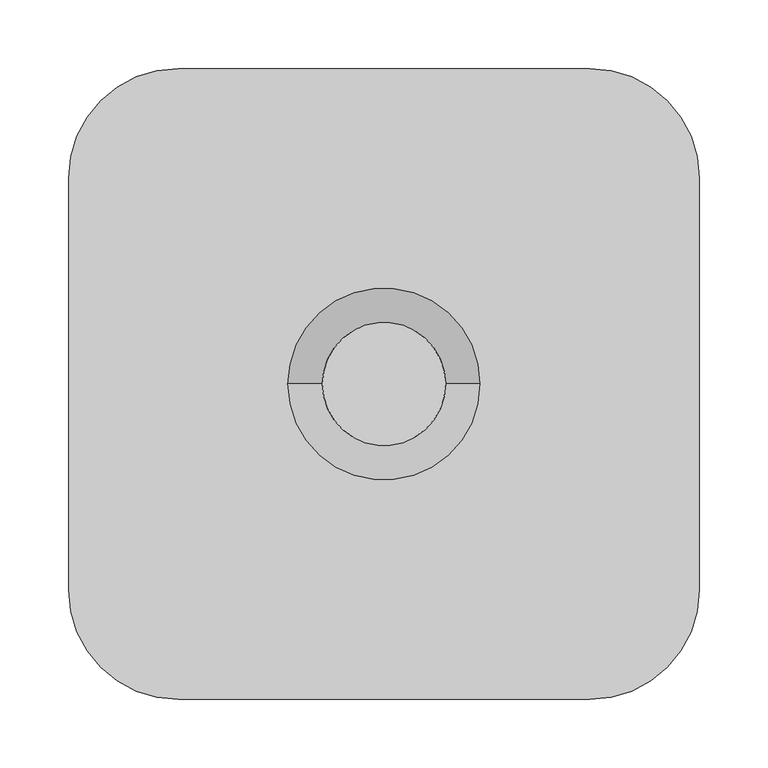
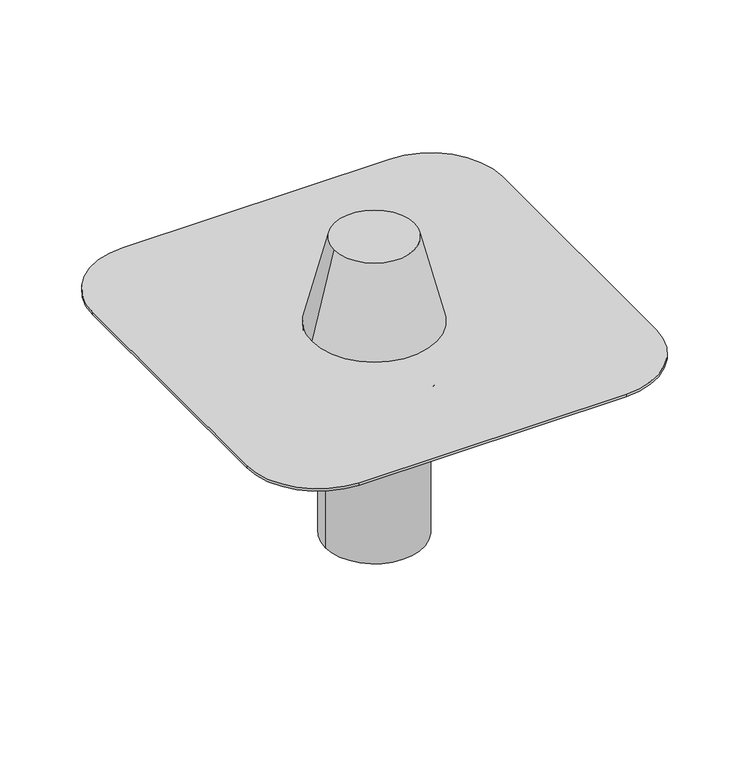
"""IFC4 building model written with IfcOpenShell, lengths in millimetres: proxy geometry, TN_ПВХ Воронка экструдированная с листоуловителем : ПВХ Воронка экструдированная 110х240мм с листоуловителем."""

import ifcopenshell
import ifcopenshell.guid

model = None  # the IFC model being written
_history = None  # IfcOwnerHistory: only IFC2X3 demands one
_inside = {}  # id of a spatial element -> (the spatial element, [elements in it])
_under = {}  # id of a project, library or spatial element -> (it, [spatial elements below it])
_declared = {}  # id of a project -> (the project, [libraries it declares])
_typed = {}  # id of a type object -> (the type object, [elements of that type])
_made_of = {}  # id of a material, layer set ... -> (it, [elements and type objects made of it])


def new_model(schema):
    """Start an empty IFC model of exactly this schema.

    Asked for "IFC4X3", IfcOpenShell would pick the latest addendum, in which some entities
    have other attributes; the version numbers below select the first issue.
    IFC2X3 requires an IfcOwnerHistory on every rooted entity: one is made here for all.
    """
    global model, _history
    if schema == "IFC4X3":
        model = ifcopenshell.file(schema_version=(4, 3, 0, 0))
    else:
        model = ifcopenshell.file(schema=schema)
    _inside.clear()
    _under.clear()
    _declared.clear()
    _typed.clear()
    _made_of.clear()
    _history = None
    if model.schema == "IFC2X3":
        org = make("IfcOrganization", Name="unknown")
        user = make(
            "IfcPersonAndOrganization",
            ThePerson=make("IfcPerson", FamilyName="unknown"),
            TheOrganization=org,
        )
        app = make(
            "IfcApplication",
            ApplicationDeveloper=org,
            Version="unknown",
            ApplicationFullName="unknown",
            ApplicationIdentifier="unknown",
        )
        _history = make(
            "IfcOwnerHistory",
            OwningUser=user,
            OwningApplication=app,
            ChangeAction="ADDED",
            CreationDate=0,
        )
    return model


def make(cls, **values):
    """One entity of the class cls with the attributes given. An attribute that is None is left unset."""
    return model.create_entity(
        cls, **{name: value for name, value in values.items() if value is not None}
    )


def rooted(cls, **values):
    """An entity with a GlobalId (a new one), such as an element, a storey or a relation."""
    return make(cls, GlobalId=ifcopenshell.guid.new(), OwnerHistory=_history, **values)


def si_unit(unit_type, name, prefix=None):
    """IfcSIUnit, for example si_unit("LENGTHUNIT", "METRE", prefix="MILLI")."""
    return make("IfcSIUnit", UnitType=unit_type, Prefix=prefix, Name=name)


def assignment(units):
    """IfcUnitAssignment: the units of a project."""
    return None if units is None else make("IfcUnitAssignment", Units=units)


def point(xyz):
    """IfcCartesianPoint."""
    return None if xyz is None else make("IfcCartesianPoint", Coordinates=xyz)


def direction(xyz):
    """IfcDirection."""
    return None if xyz is None else make("IfcDirection", DirectionRatios=xyz)


def frame(location, z_axis=None, x_axis=None):
    """IfcAxis2Placement3D, a coordinate frame: its origin and axes. An axis left out is left unset."""
    return make(
        "IfcAxis2Placement3D",
        Location=point(location),
        Axis=direction(z_axis),
        RefDirection=direction(x_axis),
    )


def frame_2d(location, x_axis=None):
    """IfcAxis2Placement2D, a coordinate frame in the plane: its origin and x axis."""
    return make(
        "IfcAxis2Placement2D", Location=point(location), RefDirection=direction(x_axis)
    )


def origin():
    """The frame at (0, 0, 0) with its axes left unset."""
    return frame((0.0, 0.0, 0.0))


def origin_2d():
    """The frame at (0, 0) in the plane with its x axis left unset."""
    return frame_2d((0.0, 0.0))


def place(relative_to, where):
    """IfcLocalPlacement: puts the frame where relative to a parent placement (None: the world)."""
    return make(
        "IfcLocalPlacement", PlacementRelTo=relative_to, RelativePlacement=where
    )


def context(
    kind, dimensions, precision=None, world=None, true_north=None, identifier=None
):
    """IfcGeometricRepresentationContext, for example the 3D "Model" context."""
    return make(
        "IfcGeometricRepresentationContext",
        ContextIdentifier=identifier,
        ContextType=kind,
        CoordinateSpaceDimension=dimensions,
        Precision=precision,
        WorldCoordinateSystem=world,
        TrueNorth=true_north,
    )


def project(units=None, contexts=None):
    """IfcProject with its units and contexts."""
    return rooted(
        "IfcProject",
        Name="project",
        RepresentationContexts=contexts,
        UnitsInContext=assignment(units),
    )


def spatial(cls, under=None, at=None, **own):
    """A site, building, storey or space (cls), placed at a placement, below another one or the project."""
    s = rooted(cls, ObjectPlacement=at, **own)
    if under is not None:
        _under.setdefault(under.id(), (under, []))[1].append(s)
    return s


def polyline(points):
    """IfcPolyline through the points."""
    return make("IfcPolyline", Points=[point(p) for p in points])


def circle_curve(where, radius):
    """IfcCircle in the frame where."""
    return make("IfcCircle", Position=where, Radius=radius)


def trimmed(basis, trim1, trim2, sense, master):
    """IfcTrimmedCurve: the piece of a basis curve between two trims."""
    return make(
        "IfcTrimmedCurve",
        BasisCurve=basis,
        Trim1=trim1,
        Trim2=trim2,
        SenseAgreement=sense,
        MasterRepresentation=master,
    )


def segment(curve, same_sense, transition):
    """IfcCompositeCurveSegment."""
    return make(
        "IfcCompositeCurveSegment",
        Transition=transition,
        SameSense=same_sense,
        ParentCurve=curve,
    )


def composite_curve(segments, self_intersect=None):
    """IfcCompositeCurve: segments joined end to end."""
    return make("IfcCompositeCurve", Segments=segments, SelfIntersect=self_intersect)


def outline(outer, holes=None, kind="AREA"):
    """IfcArbitraryClosedProfileDef: a profile drawn as a closed curve; with holes, ...WithVoids."""
    if holes is None:
        return make("IfcArbitraryClosedProfileDef", ProfileType=kind, OuterCurve=outer)
    return make(
        "IfcArbitraryProfileDefWithVoids",
        ProfileType=kind,
        OuterCurve=outer,
        InnerCurves=holes,
    )


def extrude(swept, where, along, depth):
    """IfcExtrudedAreaSolid: the profile swept, set in the frame where, extruded along a direction by depth."""
    return make(
        "IfcExtrudedAreaSolid",
        SweptArea=swept,
        Position=where,
        ExtrudedDirection=direction(along),
        Depth=depth,
    )


def shape(context_of_items, identifier, shape_type, items):
    """IfcShapeRepresentation: the items that make up one representation, for example the "Body"."""
    return make(
        "IfcShapeRepresentation",
        ContextOfItems=context_of_items,
        RepresentationIdentifier=identifier,
        RepresentationType=shape_type,
        Items=items,
    )


def source(mapping_origin, context_of_items, identifier, shape_type, items):
    """IfcRepresentationMap: a shape defined once, which mapped items show again and again."""
    return make(
        "IfcRepresentationMap",
        MappingOrigin=mapping_origin,
        MappedRepresentation=shape(context_of_items, identifier, shape_type, items),
    )


def transform(
    local_origin,
    x_axis=None,
    y_axis=None,
    z_axis=None,
    scale=None,
    scale2=None,
    scale3=None,
    uniform=True,
):
    """IfcCartesianTransformationOperator3D, or its non-uniform kind. x_axis, y_axis, z_axis: its Axis1, 2, 3."""
    if uniform:
        return make(
            "IfcCartesianTransformationOperator3D",
            Axis1=direction(x_axis),
            Axis2=direction(y_axis),
            LocalOrigin=point(local_origin),
            Scale=scale,
            Axis3=direction(z_axis),
        )
    return make(
        "IfcCartesianTransformationOperator3DnonUniform",
        Axis1=direction(x_axis),
        Axis2=direction(y_axis),
        LocalOrigin=point(local_origin),
        Scale=scale,
        Axis3=direction(z_axis),
        Scale2=scale2,
        Scale3=scale3,
    )


def mapped(mapping_source, mapping_target):
    """IfcMappedItem: shows the shape of a source again, moved by a transform."""
    return make(
        "IfcMappedItem", MappingSource=mapping_source, MappingTarget=mapping_target
    )


def made_of(thing, what):
    """Note that an element or type object is made of a material, layer set ...; save() writes the relation."""
    if what is not None:
        _made_of.setdefault(what.id(), (what, []))[1].append(thing)
    return thing


def element(
    cls,
    number,
    at=None,
    inside=None,
    cuts=None,
    type_object=None,
    material=None,
    context=None,
    identifier="Body",
    shape_type=None,
    held_by="IfcProductDefinitionShape",
    body=None,
    shapes=None,
    **own,
):
    """One element of the class cls, such as IfcWall. Its Tag is "e" and its number.

    at: its placement. inside: the storey or other place that contains it. cuts: it is an
    opening in that element (IfcRelVoidsElement). A single representation is given by context,
    identifier, shape_type and body (its items); several are given by shapes. held_by: the class
    of the entity that holds the representations. save() writes the other relations.
    """
    e = rooted(cls, Tag="e%d" % number, ObjectPlacement=at, **own)
    if body is not None:
        shapes = [shape(context, identifier, shape_type, body)]
    if shapes is not None:
        e.Representation = make(held_by, Representations=shapes)
    if inside is not None:
        _inside.setdefault(inside.id(), (inside, []))[1].append(e)
    if cuts is not None:
        rooted(
            "IfcRelVoidsElement", RelatingBuildingElement=cuts, RelatedOpeningElement=e
        )
    if type_object is not None:
        _typed.setdefault(type_object.id(), (type_object, []))[1].append(e)
    return made_of(e, material)


def aggregate(whole, parts):
    """IfcRelAggregates: a whole, such as a stair, and the parts it consists of."""
    return rooted("IfcRelAggregates", RelatingObject=whole, RelatedObjects=parts)


def save(model, path):
    """Write the relations noted so far, then the file.

    IfcRelAggregates (storeys below a building ...), IfcRelContainedInSpatialStructure (elements
    in a storey), IfcRelDefinesByType, IfcRelAssociatesMaterial and IfcRelDeclares: one each for
    every whole, place, type object, material and project.
    """
    for whole, parts in _under.values():
        aggregate(whole, parts)
    for where, things in _inside.values():
        rooted(
            "IfcRelContainedInSpatialStructure",
            RelatedElements=things,
            RelatingStructure=where,
        )
    for kind, things in _typed.values():
        rooted("IfcRelDefinesByType", RelatedObjects=things, RelatingType=kind)
    for what, things in _made_of.values():
        rooted("IfcRelAssociatesMaterial", RelatedObjects=things, RelatingMaterial=what)
    for by, libraries in _declared.values():
        rooted("IfcRelDeclares", RelatingContext=by, RelatedDefinitions=libraries)
    model.write(path)


def plane_surface(at):
    """IfcPlane: the flat surface through the origin of the frame at, square to its z axis."""
    return make("IfcPlane", Position=at)


def revolved_surface(curve, axis_point, axis_direction):
    """IfcSurfaceOfRevolution: the curve turned about the line through axis_point along axis_direction."""
    return make(
        "IfcSurfaceOfRevolution",
        SweptCurve=make("IfcArbitraryOpenProfileDef", ProfileType="CURVE", Curve=curve),
        AxisPosition=make("IfcAxis1Placement", Location=point(axis_point), Axis=direction(axis_direction)),
    )


def advanced_brep(points, edges, surfaces, faces):
    """IfcAdvancedBrep: a solid bounded by faces that lie on surfaces and meet in shared edges.

    An edge is (start, end): straight between two places in points (the first is 0);
    or (start, end, curve); or (start, end, curve, False) where it runs against its curve.
    A face is (place in surfaces, loops), or (place, loops, False) where it looks against
    its surface's normal. A loop lists edges by number (the first is 1), with a minus sign
    where the edge is run from its end to its start. The first loop is the outer one.
    """
    corners = [point(p) for p in points]
    vertices = [make("IfcVertexPoint", VertexGeometry=c) for c in corners]
    made = []
    for start, end, *more in edges:
        made.append(
            make(
                "IfcEdgeCurve",
                EdgeStart=vertices[start],
                EdgeEnd=vertices[end],
                EdgeGeometry=more[0] if more else make("IfcPolyline", Points=[corners[start], corners[end]]),
                SameSense=more[1] if len(more) > 1 else True,
            )
        )
    hull = []
    for where, loops, *sense in faces:
        bounds = []
        for j, loop in enumerate(loops):
            ring = [make("IfcOrientedEdge", EdgeElement=made[abs(k) - 1], Orientation=k > 0) for k in loop]
            bounds.append(
                make(
                    "IfcFaceOuterBound" if j == 0 else "IfcFaceBound",
                    Bound=make("IfcEdgeLoop", EdgeList=ring),
                    Orientation=True,
                )
            )
        hull.append(make("IfcAdvancedFace", Bounds=bounds, FaceSurface=surfaces[where], SameSense=sense[0] if sense else True))
    return make("IfcAdvancedBrep", Outer=make("IfcClosedShell", CfsFaces=hull))


def specialty_equipment_c9287ae0(model_context):
    return source(origin(), model_context, "Body", "SolidModel", [
        advanced_brep(
        [(70.0, 0.0, -50.0), (-70.0, 0.0, -50.0), (55.0, 0.0, -70.0), (-55.0, 0.0, -70.0)],
        [
            (0, 1, circle_curve(frame((0.0, 0.0, -50.0), z_axis=(0.0, 0.0, 1.0), x_axis=(1.0, 0.0, 0.0)), 70.0)),
            (1, 0, circle_curve(frame((0.0, 0.0, -50.0), z_axis=(0.0, 0.0, 1.0), x_axis=(-1.0, 0.0, 0.0)), 70.0)),
            (2, 3, circle_curve(frame((0.0, 0.0, -70.0), z_axis=(0.0, 0.0, -1.0), x_axis=(-1.0, 0.0, 0.0)), 55.0)),
            (3, 2, circle_curve(frame((0.0, 0.0, -70.0), z_axis=(0.0, 0.0, -1.0), x_axis=(1.0, 0.0, 0.0)), 55.0)),
            (3, 1),
            (0, 2),
        ],
        [
            plane_surface(frame((0.0, 0.0, -50.0), z_axis=(0.0, 0.0, 1.0), x_axis=(0.0, 1.0, 0.0))),
            plane_surface(frame((0.0, 0.0, -70.0), z_axis=(0.0, 0.0, -1.0), x_axis=(0.0, 1.0, 0.0))),
            revolved_surface(polyline([(-54.99999999464286, 0.0, -70.0), (-70.0, 0.0, -50.0)]), (0.0, 0.0, -143.3333333), (0.0, 0.0, 1.0)),
            revolved_surface(polyline([(54.99999999464286, 0.0, -70.0), (70.0, 0.0, -50.0)]), (0.0, 0.0, -143.3333333), (0.0, 0.0, 1.0)),
        ],
        [
            (0, [[1, 2]]),
            (1, [[3, 4]]),
            (2, [[-4, 5, -1, 6]]),
            (3, [[-3, -6, -2, -5]]),
        ],
    ),
        extrude(outline(composite_curve([segment(trimmed(circle_curve(origin_2d(), 70.0), [point((-70.0, 0.0))], [point((70.0, 0.0))], False, "CARTESIAN"), True, "CONTINUOUS"), segment(trimmed(circle_curve(origin_2d(), 70.0), [point((70.0, 0.0))], [point((-70.0, 0.0))], False, "CARTESIAN"), True, "CONTINUOUS")], self_intersect=False)), frame((0.0, 0.0, -50.0), z_axis=(0.0, 0.0, 1.0), x_axis=(1.0, 0.0, 0.0)), (0.0, 0.0, 1.0), 47.0),
        extrude(outline(composite_curve([segment(trimmed(circle_curve(origin_2d(), 55.0), [point((55.0, 0.0))], [point((-55.0, 0.0))], False, "CARTESIAN"), True, "CONTINUOUS"), segment(trimmed(circle_curve(origin_2d(), 55.0), [point((-55.0, 0.0))], [point((55.0, 0.0))], False, "CARTESIAN"), True, "CONTINUOUS")], self_intersect=False)), frame((0.0, 0.0, -250.0), z_axis=(0.0, 0.0, 1.0), x_axis=(1.0, 0.0, 0.0)), (0.0, 0.0, 1.0), 180.0),
        advanced_brep(
        [(-45.0, 0.0, 100.0), (45.0, 0.0, 100.0), (-70.0, 0.0, 0.0), (70.0, 0.0, 0.0)],
        [
            (0, 1, circle_curve(frame((0.0, 0.0, 100.0), z_axis=(0.0, 0.0, 1.0), x_axis=(-1.0, 0.0, 0.0)), 45.0)),
            (1, 0, circle_curve(frame((0.0, 0.0, 100.0), z_axis=(0.0, 0.0, 1.0), x_axis=(1.0, 0.0, 0.0)), 45.0)),
            (2, 3, circle_curve(frame((0.0, 0.0, 0.0), z_axis=(0.0, 0.0, -1.0), x_axis=(1.0, 0.0, 0.0)), 70.0)),
            (3, 2, circle_curve(frame((0.0, 0.0, 0.0), z_axis=(0.0, 0.0, -1.0), x_axis=(-1.0, 0.0, 0.0)), 70.0)),
            (3, 1),
            (0, 2),
        ],
        [
            plane_surface(frame((0.0, 0.0, 100.0), z_axis=(0.0, 0.0, 1.0), x_axis=(0.0, -1.0, 0.0))),
            plane_surface(frame((0.0, 0.0, 0.0), z_axis=(0.0, 0.0, -1.0), x_axis=(0.0, -1.0, 0.0))),
            revolved_surface(polyline([(-45.0, 0.0, 100.0), (-70.0, 0.0, 0.0)]), (0.0, 0.0, 280.0), (0.0, 0.0, -1.0)),
            revolved_surface(polyline([(45.0, 0.0, 100.0), (70.0, 0.0, 0.0)]), (0.0, 0.0, 280.0), (0.0, 0.0, -1.0)),
        ],
        [
            (0, [[1, 2]]),
            (1, [[3, 4]]),
            (2, [[-4, 5, -1, 6]]),
            (3, [[-3, -6, -2, -5]]),
        ],
    ),
        extrude(outline(composite_curve([segment(trimmed(circle_curve(frame_2d((150.0, 150.0)), 80.0), [point((150.0, 230.0))], [point((230.0, 150.0))], False, "CARTESIAN"), True, "CONTINUOUS"), segment(polyline([(230.0, 150.0), (230.0, -150.0)]), True, "CONTINUOUS"), segment(trimmed(circle_curve(frame_2d((150.0, -150.0)), 80.0), [point((230.0, -150.0))], [point((150.0, -230.0))], False, "CARTESIAN"), True, "CONTINUOUS"), segment(polyline([(150.0, -230.0), (-150.0, -230.0)]), True, "CONTINUOUS"), segment(trimmed(circle_curve(frame_2d((-150.0, -150.0)), 80.0), [point((-150.0, -230.0))], [point((-230.0, -150.0))], False, "CARTESIAN"), True, "CONTINUOUS"), segment(polyline([(-230.0, -150.0), (-230.0, 150.0)]), True, "CONTINUOUS"), segment(trimmed(circle_curve(frame_2d((-150.0, 150.0)), 80.0), [point((-230.0, 150.0))], [point((-150.0, 230.0))], False, "CARTESIAN"), True, "CONTINUOUS"), segment(polyline([(-150.0, 230.0), (150.0, 230.0)]), True, "CONTINUOUS")], self_intersect=False)), frame((0.0, 0.0, -3.0), z_axis=(0.0, 0.0, 1.0), x_axis=(1.0, 0.0, 0.0)), (0.0, 0.0, 1.0), 3.0),
    ])


if __name__ == "__main__":
    model = new_model("IFC4")
    model_context = context("Model", 3, world=origin())
    ifc_project = project(units=[si_unit("LENGTHUNIT", "METRE", prefix="MILLI")], contexts=[model_context])
    site = spatial("IfcSite", under=ifc_project)
    building = spatial("IfcBuilding", under=site)
    placement = place(None, origin())
    specialty_equipment_shape = specialty_equipment_c9287ae0(model_context)
    element("IfcBuildingElementProxy", 1, Name="TN_ПВХ Воронка экструдированная с листоуловителем : ПВХ Воронка экструдированная 110х240мм с листоуловителем", ObjectType="TN_ПВХ Воронка экструдированная с листоуловителем : ПВХ Воронка экструдированная 110х240мм с листоуловителем", at=placement, inside=building, context=model_context, shape_type="MappedRepresentation", body=[
        mapped(specialty_equipment_shape, transform((0.0, 0.0, 0.0), x_axis=(1.0, 0.0, 0.0), y_axis=(0.0, 1.0, 0.0), z_axis=(0.0, 0.0, 1.0))),
    ])
    save(model, "model.ifc")

# Revit data of these elements
# Type "TN_ПВХ Воронка экструдированная с листоуловителем : ПВХ Воронка экструдированная 110х240мм с листоуловителем"
#   ADSK_Группирование = "Комплектующие и воронки"
#   Description = "Экструдированная ПВХ воронка 110х240мм ТехноНИКОЛЬ – кровельная воронка с листвоуловителем применяется совместно с ПВХ мембранами LOGICROOF и ECOPLAST. Приваривается к мембране гомогенно при помощи горячего воздуха. Масса 600 г."
#   Manufacturer = "ТехноНИКОЛЬ"
#   URL = "http://nav.tn.ru/catalog/krovlya/vodostochnaya-sistema/pvkh-voronka-ekstrudirovannaya-tekhnonikol/?sphrase_id=42608"
#   ADSK_Примечание = ""
#   ADSK_Обозначение = "ТехноНИКОЛЬ"
#   ADSK_Наименование = "ПВХ Воронка экструдированная 110х240мм с листоуловителем"
#   ADSK_Марка = ""
#   ADSK_Код изделия = "346432"
#   ADSK_Завод-изготовитель = "ТехноНИКОЛЬ"
#   ADSK_Единица измерения = "шт."
#   ADSK_Группирование = "Комплектующие и воронки"
#   ADSK_URL страницы изделия = "https://shop.tn.ru/pvh-voronka-jekstrudirovannaja-110h240-mm"
#   ADSK_URL документации изделия = "https://nav.tn.ru/upload/iblock/8ec/Tekhlist-7.50_PVKH-voronka-ekstrudirovannaya_rus.pdf"
#   Радиус воронки низ = 55 mm
#   Радиус воронки верх = 70 mm
#   Default Elevation = 1219.2 mm
#   Длина расчетная [instance default] = 250 mm
#   Длина отвода [instance default] = 250 mm
#   Диаметр защитной решетки низ = 140 mm
#   Диаметр защитной решетки верх = 90 mm
#   Диаметр воронки низ = 110 mm
#   Диаметр воронки верх = 140 mm
#   ADSK_Масса = 0.73
#   ADSK_Количество = 1
#   Материал B = TN_ПВХ_Черный
#   Материал A = TN_ПВХ_Серый
# Element 1 (IfcBuildingElementProxy, "TN_ПВХ Воронка экструдированная с листоуловителем : ПВХ Воронка экструдированная 110х240мм с листоуловителем")
#   Materials on its faces: "TN_ПВХ_Серый", "TN_ПВХ_Черный"
# Materials
#   "TN_ПВХ_Черный": class "Типовые", colour RGB 48 48 48, transparency 0, Cost = 0
#   "TN_ПВХ_Серый": class "Типовые", colour RGB 192 192 192, transparency 0, Cost = 0
